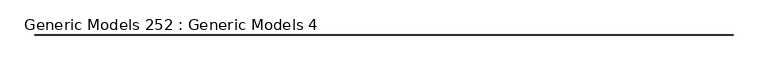
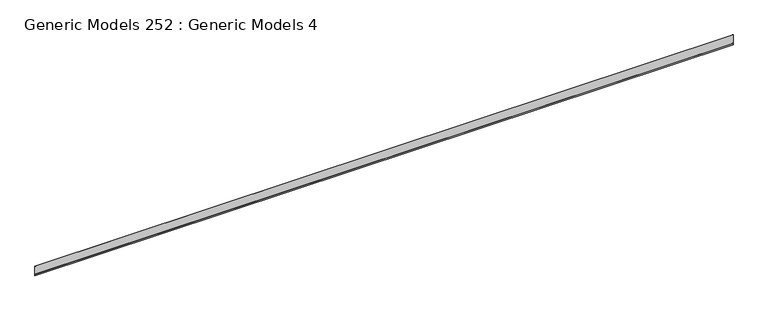
"""IFC4 building model written with IfcOpenShell, lengths in millimetres: proxy geometry, Generic Models 252 : Generic Models 4."""

from ifc_helpers import new_model, si_unit, frame, origin, place, context, project, spatial, polyline, outline, extrude, source, transform, mapped, element, save


def generic_models_252_generic_models_4_68440029(model_context):
    return source(origin(), model_context, "Body", "SweptSolid", [
        extrude(outline(polyline([(11504.6509053, 127044.7938468), (11502.0550912, 127051.9257873), (11502.0550912, 127283.615647), (11502.8488412, 127283.615647), (11502.8488412, 127052.0657468), (11505.4446553, 127044.9338063), (11505.4446553, 127005.543203), (11504.6509053, 127005.543203), (11504.6509053, 127044.7938468)])), frame((-10234.5171316, 0.0, 0.0), z_axis=(1.0, 0.0, 0.0), x_axis=(0.0, 1.0, 0.0)), (0.0, 0.0, 1.0), 18643.6),
    ])


if __name__ == "__main__":
    model = new_model("IFC4")
    model_context = context("Model", 3, world=origin())
    ifc_project = project(units=[si_unit("LENGTHUNIT", "METRE", prefix="MILLI")], contexts=[model_context])
    site = spatial("IfcSite", under=ifc_project)
    building = spatial("IfcBuilding", under=site)
    placement = place(None, origin())
    generic_models_252_generic_models_4_shape = generic_models_252_generic_models_4_68440029(model_context)
    element("IfcBuildingElementProxy", 1, Name="Generic Models 252 : Generic Models 4", ObjectType="Generic Models 252 : Generic Models 4", at=placement, inside=building, context=model_context, shape_type="MappedRepresentation", body=[
        mapped(generic_models_252_generic_models_4_shape, transform((0.0, 0.0, 0.0), x_axis=(1.0, 0.0, 0.0), y_axis=(0.0, 1.0, 0.0), z_axis=(0.0, 0.0, 1.0))),
    ])
    save(model, "model.ifc")

# Revit data of these elements
# Element 1 (IfcBuildingElementProxy, "Generic Models 252 : Generic Models 4")
#   Materials on its faces: "_(2) LAYERS NO. 30 ASTM D226 ASPHALT SATURATED ORGANIC FELT"
# Materials
#   "_(2) LAYERS NO. 30 ASTM D226 ASPHALT SATURATED ORGANIC FELT": class "Generic", colour RGB 67 154 161, transparency 0, Cost = 0
